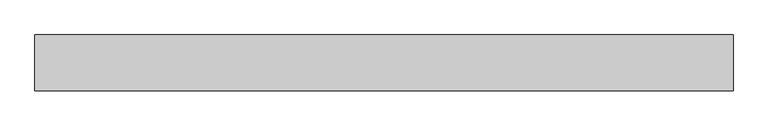
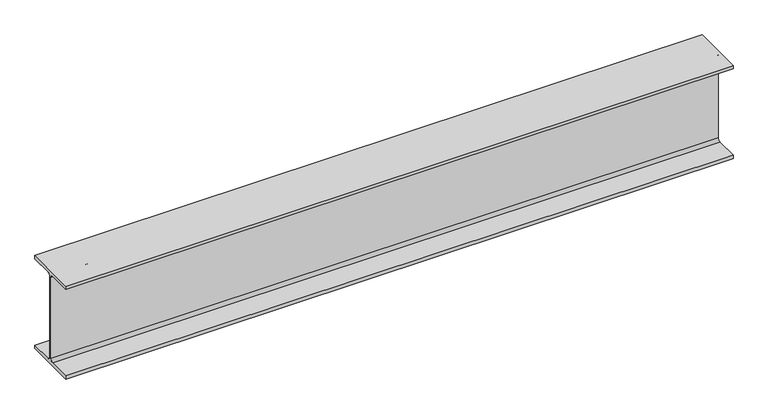
"""IFC4 building model written with IfcOpenShell, lengths in millimetres: beam geometry, Old_Steel Beam_H-KSD3502 : H_SB_ASB_H-194×150x6x9."""

from ifc_helpers import new_model, si_unit, point, frame, frame_2d, origin, place, context, project, spatial, polyline, circle_curve, trimmed, segment, composite_curve, outline, extrude, source, transform, mapped, element, save


def beam_4e962ed0(model_context):
    return source(origin(), model_context, "Body", "SweptSolid", [
        extrude(outline(composite_curve([segment(polyline([(82.5, -141.5), (82.5, -151.7), (-82.5, -151.7), (-82.5, -141.5), (-11.9, -141.5)]), True, "CONTINUOUS"), segment(trimmed(circle_curve(frame_2d((-11.9, -132.6)), 8.9), [point((-11.9, -141.5))], [point((-3.0, -132.6))], True, "CARTESIAN"), True, "CONTINUOUS"), segment(polyline([(-3.0, -132.6), (-3.0, 132.6)]), True, "CONTINUOUS"), segment(trimmed(circle_curve(frame_2d((-11.9, 132.6)), 8.9), [point((-3.0, 132.6))], [point((-11.9, 141.5))], True, "CARTESIAN"), True, "CONTINUOUS"), segment(polyline([(-11.9, 141.5), (-82.5, 141.5), (-82.5, 151.7), (82.5, 151.7), (82.5, 141.5), (11.9, 141.5)]), True, "CONTINUOUS"), segment(trimmed(circle_curve(frame_2d((11.9, 132.6)), 8.9), [point((11.9, 141.5))], [point((3.0, 132.6))], True, "CARTESIAN"), True, "CONTINUOUS"), segment(polyline([(3.0, 132.6), (3.0, -132.6)]), True, "CONTINUOUS"), segment(trimmed(circle_curve(frame_2d((11.9, -132.6)), 8.9), [point((3.0, -132.6))], [point((11.9, -141.5))], True, "CARTESIAN"), True, "CONTINUOUS"), segment(polyline([(11.9, -141.5), (82.5, -141.5)]), True, "CONTINUOUS")], self_intersect=False)), frame((-1171.2564634, 0.0, 0.0), z_axis=(1.0, 0.0, 0.0), x_axis=(0.0, 1.0, 0.0)), (0.0, 0.0, 1.0), 2060.1030758),
    ])


if __name__ == "__main__":
    model = new_model("IFC4")
    model_context = context("Model", 3, world=origin())
    ifc_project = project(units=[si_unit("LENGTHUNIT", "METRE", prefix="MILLI")], contexts=[model_context])
    site = spatial("IfcSite", under=ifc_project)
    building = spatial("IfcBuilding", under=site)
    placement = place(None, origin())
    beam_shape = beam_4e962ed0(model_context)
    element("IfcBeam", 1, ObjectType="Old_Steel Beam_H-KSD3502 : H_SB_ASB_H-194×150x6x9", at=placement, inside=building, context=model_context, shape_type="MappedRepresentation", body=[
        mapped(beam_shape, transform((0.0, 0.0, 0.0), x_axis=(1.0, 0.0, 0.0), y_axis=(0.0, 1.0, 0.0), z_axis=(0.0, 0.0, 1.0))),
    ])
    save(model, "model.ifc")

# Revit data of these elements
# Type "Old_Steel Beam_H-KSD3502 : H_SB_ASB_H-194×150x6x9"
#   Width = 15.0 cm
#   Web Thickness = 0.6 cm
#   Web Fillet = 1.3 cm
#   Warping Constant = 43316.0 cm⁶
#   Torsional Moment of Inertia = 8.622 cm⁴
#   Torsional Modulus = 1.0 cm³
#   Section Area = 39.01 cm²
#   Plastic Modulus weak axis = 104.0 cm³
#   Plastic Modulus strong axis = 309.0 cm³
#   Perimeter = 0.95 m²/m
#   Nominal Weight = 30.60 kgf/m
#   Moment of Inertia weak axis = 507.00 cm⁴
#   Moment of Inertia strong axis = 2690.00 cm⁴
#   Height = 19.4 cm
#   Flange Thickness = 0.9 cm
#   Elastic Modulus weak axis = 67.6 cm³
#   Elastic Modulus strong axis = 277.0 cm³
#   Centroid Vertical = 9.7 cm
#   Centroid Horizontal = 7.5 cm
#   Length [instance default] = 1.5240 m
#   Structural Material [instance default] = Steel, 45-345
#   Assembly Code = ""
# Element 1 (IfcBeam, "Old_Steel Beam_H-KSD3502 : H_SB_ASB_H-194×150x6x9")
#   Structural Material = none
# Materials
#   "Steel, 45-345": class "Metal", colour RGB 189 187 185, transparency 0, Description = "Steel 345 MPa", Cost = 0
